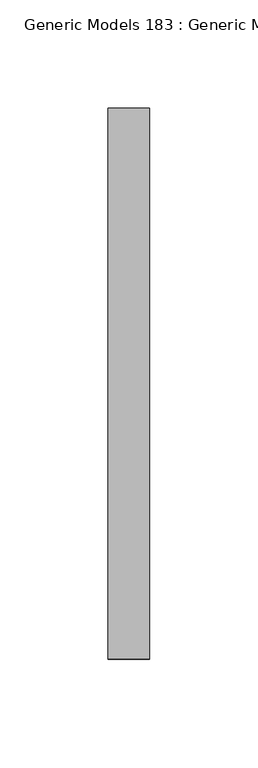
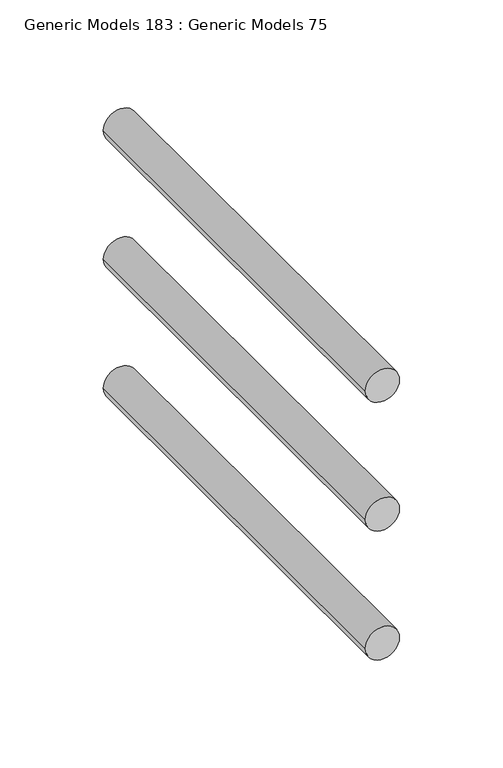
"""IFC4 building model written with IfcOpenShell, lengths in millimetres: proxy geometry, Generic Models 183 : Generic Models 75."""

from ifc_helpers import new_model, si_unit, point, frame, frame_2d, origin, place, context, project, spatial, circle_curve, trimmed, segment, composite_curve, outline, extrude, source, transform, mapped, element, save


def generic_models_183_generic_models_75_6567494b(model_context):
    return source(origin(), model_context, "Body", "SweptSolid", [
        extrude(outline(composite_curve([segment(trimmed(circle_curve(frame_2d((268976.475, 31752.3658532)), 9.525), [point((268976.475, 31742.8408532))], [point((268976.475, 31761.8908532))], False, "CARTESIAN"), True, "CONTINUOUS"), segment(trimmed(circle_curve(frame_2d((268976.475, 31752.3658532)), 9.525), [point((268976.475, 31761.8908532))], [point((268976.475, 31742.8408532))], False, "CARTESIAN"), True, "CONTINUOUS")], self_intersect=False)), frame((0.0, 30647.3406612, 0.0), z_axis=(0.0, 1.0, 0.0), x_axis=(0.0, 0.0, 1.0)), (0.0, 0.0, 1.0), 254.0),
        extrude(outline(composite_curve([segment(trimmed(circle_curve(frame_2d((268900.275, 31752.3658532)), 9.525), [point((268900.275, 31742.8408532))], [point((268900.275, 31761.8908532))], False, "CARTESIAN"), True, "CONTINUOUS"), segment(trimmed(circle_curve(frame_2d((268900.275, 31752.3658532)), 9.525), [point((268900.275, 31761.8908532))], [point((268900.275, 31742.8408532))], False, "CARTESIAN"), True, "CONTINUOUS")], self_intersect=False)), frame((0.0, 30647.3406612, 0.0), z_axis=(0.0, 1.0, 0.0), x_axis=(0.0, 0.0, 1.0)), (0.0, 0.0, 1.0), 254.0),
        extrude(outline(composite_curve([segment(trimmed(circle_curve(frame_2d((269052.675, 31752.3658532)), 9.525), [point((269052.675, 31742.8408532))], [point((269052.675, 31761.8908532))], False, "CARTESIAN"), True, "CONTINUOUS"), segment(trimmed(circle_curve(frame_2d((269052.675, 31752.3658532)), 9.525), [point((269052.675, 31761.8908532))], [point((269052.675, 31742.8408532))], False, "CARTESIAN"), True, "CONTINUOUS")], self_intersect=False)), frame((0.0, 30647.3406612, 0.0), z_axis=(0.0, 1.0, 0.0), x_axis=(0.0, 0.0, 1.0)), (0.0, 0.0, 1.0), 254.0),
    ])


if __name__ == "__main__":
    model = new_model("IFC4")
    model_context = context("Model", 3, world=origin())
    ifc_project = project(units=[si_unit("LENGTHUNIT", "METRE", prefix="MILLI")], contexts=[model_context])
    site = spatial("IfcSite", under=ifc_project)
    building = spatial("IfcBuilding", under=site)
    placement = place(None, origin())
    generic_models_183_generic_models_75_shape = generic_models_183_generic_models_75_6567494b(model_context)
    element("IfcBuildingElementProxy", 1, Name="Generic Models 183 : Generic Models 75", ObjectType="Generic Models 183 : Generic Models 75", at=placement, inside=building, context=model_context, shape_type="MappedRepresentation", body=[
        mapped(generic_models_183_generic_models_75_shape, transform((0.0, 0.0, 0.0), x_axis=(1.0, 0.0, 0.0), y_axis=(0.0, 1.0, 0.0), z_axis=(0.0, 0.0, 1.0))),
    ])
    save(model, "model.ifc")
